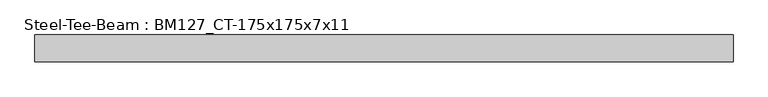
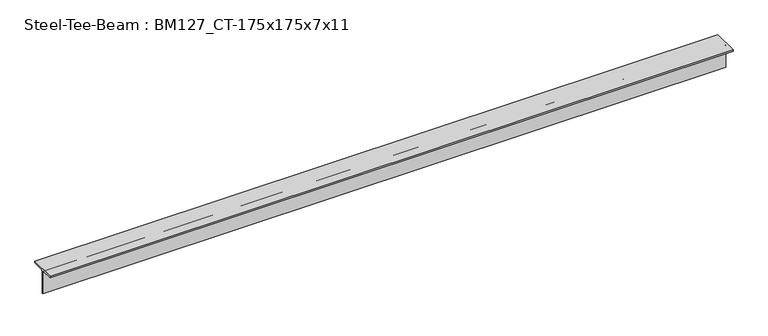
"""IFC4 building model written with IfcOpenShell, lengths in millimetres: beam geometry, Steel-Tee-Beam : BM127_CT-175x175x7x11."""

from ifc_helpers import new_model, si_unit, point, frame, frame_2d, origin, place, context, project, spatial, polyline, circle_curve, trimmed, segment, composite_curve, outline, extrude, source, transform, mapped, element, save


def steel_tee_beam_bm127_ct_175x175x7x11_4594752c(model_context):
    return source(origin(), model_context, "Body", "SweptSolid", [
        extrude(outline(composite_curve([segment(polyline([(-87.5, 87.5), (87.5, 87.5), (87.5, 76.5), (17.5, 76.5)]), True, "CONTINUOUS"), segment(trimmed(circle_curve(frame_2d((17.5, 62.5)), 14.0), [point((17.5, 76.5))], [point((3.5, 62.5))], True, "CARTESIAN"), True, "CONTINUOUS"), segment(polyline([(3.5, 62.5), (3.5, -87.5), (-3.5, -87.5), (-3.5, 62.5)]), True, "CONTINUOUS"), segment(trimmed(circle_curve(frame_2d((-17.5, 62.5)), 14.0), [point((-3.5, 62.5))], [point((-17.5, 76.5))], True, "CARTESIAN"), True, "CONTINUOUS"), segment(polyline([(-17.5, 76.5), (-87.5, 76.5), (-87.5, 87.5)]), True, "CONTINUOUS")], self_intersect=False)), frame((-2375.7579713, 0.0, 0.0), z_axis=(1.0, 0.0, 0.0), x_axis=(0.0, 1.0, 0.0)), (0.0, 0.0, 1.0), 4573.2110535),
    ])


if __name__ == "__main__":
    model = new_model("IFC4")
    model_context = context("Model", 3, world=origin())
    ifc_project = project(units=[si_unit("LENGTHUNIT", "METRE", prefix="MILLI")], contexts=[model_context])
    site = spatial("IfcSite", under=ifc_project)
    building = spatial("IfcBuilding", under=site)
    placement = place(None, origin())
    steel_tee_beam_bm127_ct_175x175x7x11_shape = steel_tee_beam_bm127_ct_175x175x7x11_4594752c(model_context)
    element("IfcBeam", 1, ObjectType="Steel-Tee-Beam : BM127_CT-175x175x7x11", at=placement, inside=building, context=model_context, shape_type="MappedRepresentation", body=[
        mapped(steel_tee_beam_bm127_ct_175x175x7x11_shape, transform((0.0, 0.0, 0.0), x_axis=(1.0, 0.0, 0.0), y_axis=(0.0, 1.0, 0.0), z_axis=(0.0, 0.0, 1.0))),
    ])
    save(model, "model.ifc")

# Revit data of these elements
# Type "Steel-Tee-Beam : BM127_CT-175x175x7x11"
#   Surface Area = 0.00 m²/m
#   Section Area = 31.57 cm²
#   Mass per Unit Length = 24.80 kg/m
#   Length [instance default] = 1524 mm
#   bf = 175 mm
#   d = 175 mm
#   k = 25 mm
#   kr = 14 mm
#   tf = 11 mm
#   tw = 7 mm
#   hec_material4 [instance default] = none
#   hec_material3 [instance default] = none
#   hec_material2 [instance default] = none
#   hec_material1 [instance default] = none
#   Structural Material [instance default] = Steel, 45-345
#   Assembly Code = ""
# Element 1 (IfcBeam, "Steel-Tee-Beam : BM127_CT-175x175x7x11")
#   hec_material3 = F01AC000-00002_Building/Shelter Fire Proofing Work_Intumescent Coating Type_1 hr. rating (UL 1709))
#   hec_material2 = S01AA010-00002_Main Steel Structure Fabrication Work_Shelter/Building_Steel Painting/Coating_for Fireproofed Steel Surface, Surface Preparation & Primer Coat
#   hec_material1 = S03AA029-00001_Main Steel Structure Erection Work_Shelter/Building_Light Steel
#   Structural Material = S01AA003-00001_Main Steel Structure Fabrication Work_Shelter/Building_Light Steel - Standard
#   Materials on its faces: "S01AA003-00001_Main Steel Structure Fabrication Work_Shelter/Building_Light Steel - Standard"
# Materials
#   "Steel, 45-345": class "Metal", colour RGB 189 187 185, transparency 0, Description = "Steel 345 MPa", Cost = 0
#   "S01AA003-00001_Main Steel Structure Fabrication Work_Shelter/Building_Light Steel - Standard": class "Metal", colour RGB 120 120 120, transparency 0, Comments = "(30KG/M>Weight)", Description = "Structural steel 50ksi", W00) Work Master Code = "S01AA003-00001", W01) Work Master_Lv1 = "Main Steel Structure Fabrication Work", W02) Work Master_Lv2 = "Shelter/Building", W03) Work Master_Spec.1 = "Light Steel - Standard (30KG/M>Weight)", Cost = 0
#   "F01AC000-00002_Building/Shelter Fire Proofing Work_Intumescent Coating Type_1 hr. rating (UL 1709))": class "Metal", colour RGB 255 128 128, transparency 0, Description = "Paint finished steel", W00) Work Master Code = "F01AC000-00002", W01) Work Master_Lv1 = "Building/Shelter Fire Proofing Work", W02) Work Master_Lv2 = "Intumescent Coating Type", W03) Work Master_Spec.1 = "1 hr. rating (UL 1709)", Cost = 0
#   "S01AA010-00002_Main Steel Structure Fabrication Work_Shelter/Building_Steel Painting/Coating_for Fireproofed Steel Surface, Surface Preparation & Primer Coat": class "Metal", colour RGB 120 120 120, transparency 0, Description = "Paint finished steel", W00) Work Master Code = "SS01AA010-00002", W01) Work Master_Lv1 = "Main Steel Structure Fabrication Work", W02) Work Master_Lv2 = "Shelter/Building", W03) Work Master_Spec.1 = "Steel Painting/Coating", W04) Work Master_Spec.2 = "for Fireproofed Steel Surface, Surface Preparation & Primer Coat", Cost = 0
#   "S03AA029-00001_Main Steel Structure Erection Work_Shelter/Building_Light Steel": class "Metal", colour RGB 120 120 120, transparency 0, Comments = "(30KG/M>Weight)", Description = "Structural steel 50ksi", W00) Work Master Code = "S03AA029-00001", W01) Work Master_Lv1 = "Main Steel Structure Erection Work", W02) Work Master_Lv2 = "Shelter/Building", W03) Work Master_Spec.1 = "Light Steel (30KG/M>Weight)", Cost = 0
